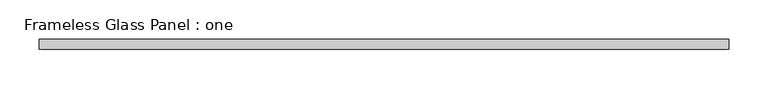
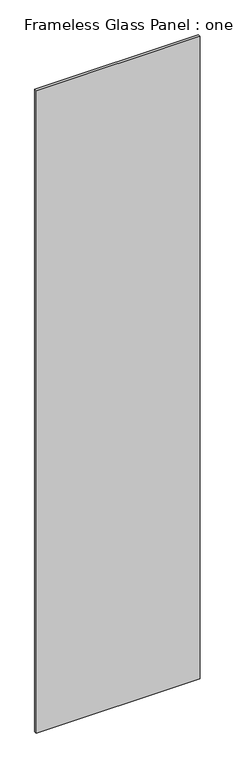
"""IFC4 building model written with IfcOpenShell, lengths in millimetres: plate geometry, Frameless Glass Panel : one."""

from ifc_helpers import new_model, si_unit, origin, origin_with_axes, place, context, project, spatial, polyline, outline, extrude, source, transform, mapped, element, save


def frameless_glass_panel_one_1c9fb1ae(model_context):
    return source(origin(), model_context, "Body", "SweptSolid", [
        extrude(outline(polyline([(440.8100761, -6.35), (-440.8100761, -6.35), (-440.8100761, 6.35), (440.8100761, 6.35), (440.8100761, -6.35)])), origin_with_axes(), (0.0, 0.0, 1.0), 3651.25),
    ])


if __name__ == "__main__":
    model = new_model("IFC4")
    model_context = context("Model", 3, world=origin())
    ifc_project = project(units=[si_unit("LENGTHUNIT", "METRE", prefix="MILLI")], contexts=[model_context])
    site = spatial("IfcSite", under=ifc_project)
    building = spatial("IfcBuilding", under=site)
    placement = place(None, origin())
    frameless_glass_panel_one_shape = frameless_glass_panel_one_1c9fb1ae(model_context)
    element("IfcPlate", 1, ObjectType="Frameless Glass Panel : one", at=placement, inside=building, context=model_context, shape_type="MappedRepresentation", body=[
        mapped(frameless_glass_panel_one_shape, transform((0.0, 0.0, 0.0), x_axis=(1.0, 0.0, 0.0), y_axis=(0.0, 1.0, 0.0), z_axis=(0.0, 0.0, 1.0))),
    ])
    save(model, "model.ifc")

# Revit data of these elements
# Type "Frameless Glass Panel : one"
#   Glass Thickness = 0' - 0 1/2"
#   Gap btwn Panels = 0' - 0 1/4"
#   Panel Material = TEMPERED GLASS DOOR/SIDELIGHT TO MATCH EXISTING CONF. ROOM
# Element 1 (IfcPlate, "Frameless Glass Panel : one")
#   Materials on its faces: "TEMPERED GLASS DOOR/SIDELIGHT TO MATCH EXISTING CONF. ROOM"
# Materials
#   "TEMPERED GLASS DOOR/SIDELIGHT TO MATCH EXISTING CONF. ROOM": class "Glass", colour RGB 218 227 224, transparency 0.85, Description = "Soda Lime Glass", Cost = 0
